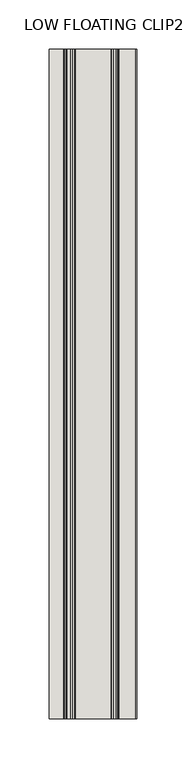
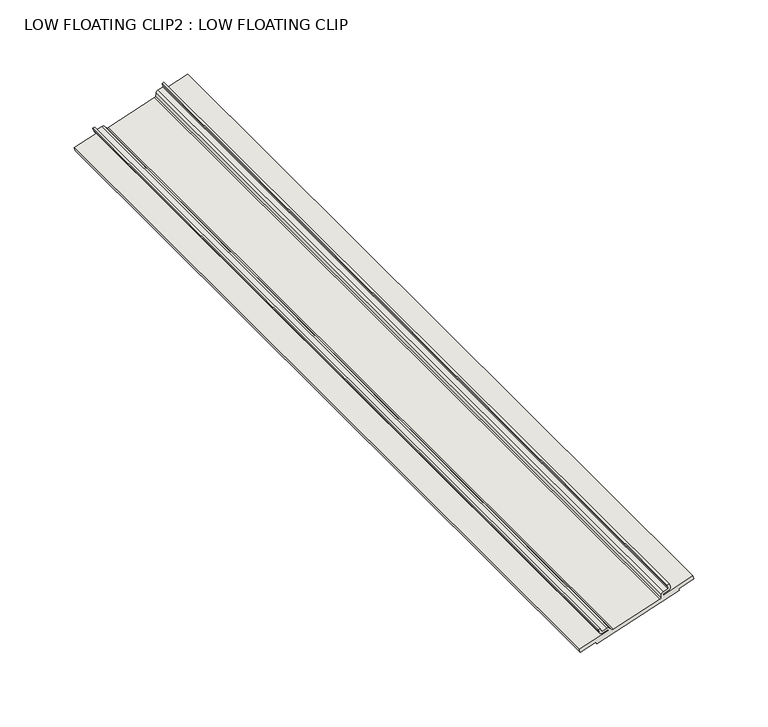
"""IFC4 building model written with IfcOpenShell, lengths in millimetres: wall geometry, LOW FLOATING CLIP2 : LOW FLOATING CLIP."""

from ifc_helpers import new_model, si_unit, frame, origin, place, context, project, spatial, polyline, circle_curve, source, transform, mapped, element, save
from ifc_brep_helpers import plane_surface, cylinder_surface, revolved_surface, advanced_brep


def low_floating_clip2_low_floating_clip_d8918f67(model_context):
    return source(origin(), model_context, "Body", "AdvancedBrep", [
        advanced_brep(
        [(21251.6963274, -2319.6634634, 5817.03297), (21250.2517072, -2319.6634634, 5816.5493228), (21251.0580869, -2319.6634634, 5814.1407232), (21250.6406207, -2319.6634634, 5813.3039581), (21247.0206876, -2319.6634634, 5812.0920337), (21245.5343092, -2319.6634634, 5810.171657), (21245.3411622, -2319.6634634, 5807.4026721), (21244.3180461, -2319.6634634, 5807.060141), (21208.189862, -2319.6634634, 5794.9647155), (21207.1667458, -2319.6634634, 5794.6221844), (21205.3453341, -2319.6634634, 5796.7167113), (21203.0023221, -2319.6634634, 5797.3550388), (21199.3823891, -2319.6634634, 5796.1431143), (21198.5458, -2319.6634634, 5796.5600318), (21197.7388807, -2319.6634634, 5798.9684507), (21196.2942605, -2319.6634634, 5798.4848035), (21197.1006403, -2319.6634634, 5796.076204), (21199.8649785, -2319.6634634, 5794.6985661), (21203.9031762, -2319.6634634, 5796.0505222), (21204.6364349, -2319.6634634, 5795.2073261), (21181.5643102, -2319.6634634, 5787.4829643), (21182.4790038, -2319.6634634, 5784.7508388), (21194.5228505, -2319.6634634, 5788.7830219), (21195.0069954, -2319.6634634, 5787.336915), (21259.436224, -2319.6634634, 5808.9073026), (21258.952079, -2319.6634634, 5810.3534096), (21270.9959257, -2319.6634634, 5814.3855926), (21270.0812321, -2319.6634634, 5817.117718), (21247.0091074, -2319.6634634, 5809.3933561), (21247.0868715, -2319.6634634, 5810.5080761), (21251.1250692, -2319.6634634, 5811.8600323), (21252.5027071, -2319.6634634, 5814.6243705), (21251.6963274, -1637.0384634, 5817.03297), (21252.5027071, -1637.0384634, 5814.6243705), (21251.1250692, -1637.0384634, 5811.8600323), (21247.0868715, -1637.0384634, 5810.5080761), (21247.0091074, -1637.0384634, 5809.3933561), (21270.0812321, -1637.0384634, 5817.117718), (21270.9959257, -1637.0384634, 5814.3855926), (21258.952079, -1637.0384634, 5810.3534096), (21259.436224, -1637.0384634, 5808.9073026), (21195.0069954, -1637.0384634, 5787.336915), (21194.5228505, -1637.0384634, 5788.7830219), (21182.4790038, -1637.0384634, 5784.7508388), (21181.5643102, -1637.0384634, 5787.4829643), (21204.6364349, -1637.0384634, 5795.2073261), (21203.9031762, -1637.0384634, 5796.0505222), (21199.8649785, -1637.0384634, 5794.6985661), (21197.1006403, -1637.0384634, 5796.076204), (21196.2942605, -1637.0384634, 5798.4848035), (21197.7388807, -1637.0384634, 5798.9684507), (21198.5452605, -1637.0384634, 5796.5598512), (21199.3823891, -1637.0384634, 5796.1431143), (21203.0023221, -1637.0384634, 5797.3550388), (21205.3453341, -1637.0384634, 5796.7167113), (21207.1667458, -1637.0384634, 5794.6221844), (21208.189862, -1637.0384634, 5794.9647155), (21244.3180461, -1637.0384634, 5807.060141), (21245.3411622, -1637.0384634, 5807.4026721), (21245.5343092, -1637.0384634, 5810.171657), (21247.0206876, -1637.0384634, 5812.0920337), (21250.6406207, -1637.0384634, 5813.3039581), (21251.0575474, -1637.0384634, 5814.1405426), (21250.2517072, -1637.0384634, 5816.5493228)],
        [
            (0, 1),
            (1, 2),
            (2, 3, circle_curve(frame((21250.4307872, -2319.6634634, 5813.930716), z_axis=(0.0, 1.0, 0.0), x_axis=(0.31747234470250746, 0.0, -0.9482675310001353)), 0.6609505)),
            (3, 4),
            (4, 5, circle_curve(frame((21247.714529, -2319.6634634, 5810.0195786), z_axis=(0.0, -1.0, 0.0), x_axis=(-0.997576050299932, 0.0, 0.06958465253191609)), 2.1855173)),
            (5, 6),
            (6, 7),
            (7, 8),
            (8, 9),
            (9, 10),
            (10, 11, circle_curve(frame((21203.6961634, -2319.6634634, 5795.2825837), z_axis=(0.0, -1.0, 0.0), x_axis=(0.7545905437642736, 0.0, 0.6561959396868727)), 2.1855173)),
            (11, 12),
            (12, 13, circle_curve(frame((21199.1725556, -2319.6634634, 5796.7698722), z_axis=(0.0, 1.0, 0.0), x_axis=(0.3174723447027873, 0.0, -0.9482675310000416)), 0.6609505)),
            (13, 14),
            (14, 15),
            (15, 16),
            (16, 17, circle_curve(frame((21199.1716283, -2319.6634634, 5796.7695541), z_axis=(0.0, -1.0, 0.0), x_axis=(-0.9482675310000763, 0.0, -0.3174723447026833)), 2.1839702)),
            (17, 18),
            (18, 19),
            (19, 20),
            (20, 21),
            (21, 22),
            (22, 23),
            (23, 24),
            (24, 25),
            (25, 26),
            (26, 27),
            (27, 28),
            (28, 29),
            (29, 30),
            (30, 31, circle_curve(frame((21250.4317191, -2319.6634634, 5813.9310203), z_axis=(0.0, -1.0, 0.0), x_axis=(0.9482675310001005, 0.0, 0.31747234470261126)), 2.1839702)),
            (31, 0),
            (32, 33),
            (33, 34, circle_curve(frame((21250.4317191, -1637.0384634, 5813.9310203), z_axis=(0.0, 1.0, 0.0), x_axis=(0.9482675310001005, 0.0, 0.31747234470261126)), 2.1839702)),
            (34, 35),
            (35, 36),
            (36, 37),
            (37, 38),
            (38, 39),
            (39, 40),
            (40, 41),
            (41, 42),
            (42, 43),
            (43, 44),
            (44, 45),
            (45, 46),
            (46, 47),
            (47, 48, circle_curve(frame((21199.1716283, -1637.0384634, 5796.7695541), z_axis=(0.0, 1.0, 0.0), x_axis=(-0.9482675310000763, 0.0, -0.3174723447026833)), 2.1839702)),
            (48, 49),
            (49, 50),
            (50, 51),
            (51, 52, circle_curve(frame((21199.1725556, -1637.0384634, 5796.7698722), z_axis=(0.0, -1.0, 0.0), x_axis=(0.3174723447027873, 0.0, -0.9482675310000416)), 0.6609505)),
            (52, 53),
            (53, 54, circle_curve(frame((21203.6961634, -1637.0384634, 5795.2825837), z_axis=(0.0, 1.0, 0.0), x_axis=(0.7545905437642736, 0.0, 0.6561959396868727)), 2.1855173)),
            (54, 55),
            (55, 56),
            (56, 57),
            (57, 58),
            (58, 59),
            (59, 60, circle_curve(frame((21247.714529, -1637.0384634, 5810.0195786), z_axis=(0.0, 1.0, 0.0), x_axis=(-0.997576050299932, 0.0, 0.06958465253191609)), 2.1855173)),
            (60, 61),
            (61, 62, circle_curve(frame((21250.4307872, -1637.0384634, 5813.930716), z_axis=(0.0, -1.0, 0.0), x_axis=(0.31747234470250746, 0.0, -0.9482675310001353)), 0.6609505)),
            (62, 63),
            (63, 32),
            (31, 33),
            (32, 0),
            (30, 34),
            (29, 35),
            (28, 36),
            (27, 37),
            (26, 38),
            (25, 39),
            (24, 40),
            (23, 41),
            (22, 42),
            (21, 43),
            (20, 44),
            (19, 45),
            (18, 46),
            (17, 47),
            (16, 48),
            (15, 49),
            (14, 50),
            (13, 51),
            (12, 52),
            (11, 53),
            (10, 54),
            (9, 55),
            (8, 56),
            (7, 57),
            (6, 58),
            (5, 59),
            (4, 60),
            (3, 61),
            (2, 62),
            (1, 63),
        ],
        [
            plane_surface(frame((21250.2511677, -2319.6634634, 5816.5491422), z_axis=(0.0, -1.0000000000000002, 0.0), x_axis=(-0.9482675310000759, 0.0, -0.3174723447026848))),
            plane_surface(frame((21250.2511677, -1637.0384634, 5816.5491422), z_axis=(0.0, 1.0000000000000002, 0.0), x_axis=(0.9482675310000759, 0.0, 0.3174723447026848))),
            plane_surface(frame((21252.5027071, -2319.6634634, 5814.6243705), z_axis=(0.9482675310001323, 0.0, 0.3174723447025162), x_axis=(0.0, 1.0, 0.0))),
            cylinder_surface(frame((21250.4317191, -1637.0384634, 5813.9310203), z_axis=(0.0, -1.0000000000000002, 0.0), x_axis=(0.9482675310001005, 0.0, 0.31747234470261126)), 2.1839702),
            plane_surface(frame((21247.0868715, -2319.6634634, 5810.5080761), z_axis=(0.3174723445422707, 0.0, -0.9482675310537811), x_axis=(0.0, 1.0, 0.0))),
            plane_surface(frame((21247.0091074, -2319.6634634, 5809.3933561), z_axis=(0.9975755390756385, 0.0, -0.06959198113252213), x_axis=(0.0, 1.0, 0.0))),
            plane_surface(frame((21270.0812321, -2319.6634634, 5817.117718), z_axis=(-0.3174723447025733, 0.0, 0.9482675310001131), x_axis=(0.0, 1.0, 0.0))),
            plane_surface(frame((21270.9959257, -2319.6634634, 5814.3855926), z_axis=(0.9482675310001432, 0.0, 0.3174723447024835), x_axis=(0.0, 1.0, 0.0))),
            plane_surface(frame((21258.952079, -2319.6634634, 5810.3534096), z_axis=(0.3174723447026279, 0.0, -0.9482675310000949), x_axis=(0.0, 1.0, 0.0))),
            plane_surface(frame((21259.436224, -2319.6634634, 5808.9073026), z_axis=(0.9482675310001084, 0.0, 0.31747234470258734), x_axis=(0.0, 1.0, 0.0))),
            plane_surface(frame((21195.0069954, -2319.6634634, 5787.336915), z_axis=(0.31747234470254, 0.0, -0.9482675310001243), x_axis=(0.0, 1.0, 0.0))),
            plane_surface(frame((21194.5228505, -2319.6634634, 5788.7830219), z_axis=(-0.9482675310005341, 0.0, -0.3174723447013159), x_axis=(0.0, 1.0, 0.0))),
            plane_surface(frame((21182.4790038, -2319.6634634, 5784.7508388), z_axis=(0.3174723447026786, 0.0, -0.9482675310000779), x_axis=(0.0, 1.0, 0.0))),
            plane_surface(frame((21181.5643102, -2319.6634634, 5787.4829643), z_axis=(-0.9482675310000674, 0.0, -0.31747234470270974), x_axis=(0.0, 1.0, 0.0))),
            plane_surface(frame((21204.6364349, -2319.6634634, 5795.2073261), z_axis=(-0.31747234470271984, 0.0, 0.9482675310000641), x_axis=(0.0, 1.0, 0.0))),
            plane_surface(frame((21203.9031762, -2319.6634634, 5796.0505222), z_axis=(-0.7545857230581579, 0.0, -0.6562014832022228), x_axis=(0.0, 1.0, 0.0))),
            plane_surface(frame((21199.8649785, -2319.6634634, 5794.6985661), z_axis=(0.3174723447025522, 0.0, -0.9482675310001202), x_axis=(0.0, 1.0, 0.0))),
            cylinder_surface(frame((21199.1716283, -1637.0384634, 5796.7695541), z_axis=(0.0, -1.0, 0.0), x_axis=(-0.9482675310000763, 0.0, -0.3174723447026833)), 2.1839702),
            plane_surface(frame((21196.2942605, -2319.6634634, 5798.4848035), z_axis=(-0.9482675309984633, 0.0, -0.31747234470750146), x_axis=(0.0, 1.0, 0.0))),
            plane_surface(frame((21197.7388807, -2319.6634634, 5798.9684507), z_axis=(-0.3174723447029016, 0.0, 0.9482675310000033), x_axis=(0.0, 1.0, 0.0))),
            plane_surface(frame((21198.5452605, -2319.6634634, 5796.5598512), z_axis=(0.9482675310001752, 0.0, 0.31747234470238783), x_axis=(0.0, 1.0, 0.0))),
            revolved_surface(polyline([(21199.382389104965, -1637.0384634, 5796.143114301251), (21199.382389104965, -2319.6634634, 5796.143114301251)]), (21199.1725556, -1637.0384634, 5796.7698722), (0.0, 1.0000000000000002, 0.0)),
            plane_surface(frame((21203.0023221, -2319.6634634, 5797.3550388), z_axis=(-0.31747234470292157, 0.0, 0.9482675309999966), x_axis=(0.0, 1.0, 0.0))),
            cylinder_surface(frame((21203.6961634, -1637.0384634, 5795.2825837), z_axis=(0.0, -1.0000000000000002, 0.0), x_axis=(0.7545905437642736, 0.0, 0.6561959396868727)), 2.1855173),
            plane_surface(frame((21207.1667458, -2319.6634634, 5794.6221844), z_axis=(0.7545905437681126, 0.0, 0.656195939682458), x_axis=(0.0, 1.0, 0.0))),
            plane_surface(frame((21208.189862, -2319.6634634, 5794.9647155), z_axis=(-0.31747234470267577, 0.0, 0.9482675310000789), x_axis=(0.0, 1.0, 0.0))),
            plane_surface(frame((21244.3180461, -2319.6634634, 5807.060141), z_axis=(-0.3174723447026769, 0.0, 0.9482675310000784), x_axis=(0.0, 1.0, 0.0))),
            plane_surface(frame((21245.3411622, -2319.6634634, 5807.4026721), z_axis=(-0.31747234470207936, 0.0, 0.9482675310002785), x_axis=(0.0, 1.0, 0.0))),
            plane_surface(frame((21245.5343092, -2319.6634634, 5810.171657), z_axis=(-0.9975760502999373, 0.0, 0.06958465253183929), x_axis=(0.0, 1.0, 0.0))),
            cylinder_surface(frame((21247.714529, -1637.0384634, 5810.0195786), z_axis=(0.0, -1.0, 0.0), x_axis=(-0.997576050299932, 0.0, 0.06958465253191609)), 2.1855173),
            plane_surface(frame((21250.6406207, -2319.6634634, 5813.3039581), z_axis=(-0.317472342372389, 0.0, 0.9482675317802401), x_axis=(0.0, 1.0, 0.0))),
            revolved_surface(polyline([(21250.640620704966, -1637.0384634, 5813.303958101252), (21250.640620704966, -2319.6634634, 5813.303958101252)]), (21250.4307872, -1637.0384634, 5813.930716), (0.0, 1.0000000000000002, 0.0)),
            plane_surface(frame((21250.2517072, -2319.6634634, 5816.5493228), z_axis=(-0.9482675310001136, 0.0, -0.3174723447025722), x_axis=(0.0, 1.0, 0.0))),
            plane_surface(frame((21251.6963274, -2319.6634634, 5817.03297), z_axis=(-0.3174723447026848, 0.0, 0.9482675310000759), x_axis=(0.0, 1.0, 0.0))),
        ],
        [
            (0, [[1, 2, 3, 4, 5, 6, 7, 8, 9, 10, 11, 12, 13, 14, 15, 16, 17, 18, 19, 20, 21, 22, 23, 24, 25, 26, 27, 28, 29, 30, 31, 32]]),
            (1, [[33, 34, 35, 36, 37, 38, 39, 40, 41, 42, 43, 44, 45, 46, 47, 48, 49, 50, 51, 52, 53, 54, 55, 56, 57, 58, 59, 60, 61, 62, 63, 64]]),
            (2, [[-32, 65, -33, 66]]),
            (3, [[-31, 67, -34, -65]]),
            (4, [[-30, 68, -35, -67]]),
            (5, [[-29, 69, -36, -68]]),
            (6, [[-28, 70, -37, -69]]),
            (7, [[-27, 71, -38, -70]]),
            (8, [[-26, 72, -39, -71]]),
            (9, [[-25, 73, -40, -72]]),
            (10, [[-24, 74, -41, -73]]),
            (11, [[-23, 75, -42, -74]]),
            (12, [[-22, 76, -43, -75]]),
            (13, [[-21, 77, -44, -76]]),
            (14, [[-20, 78, -45, -77]]),
            (15, [[-19, 79, -46, -78]]),
            (16, [[-18, 80, -47, -79]]),
            (17, [[-17, 81, -48, -80]]),
            (18, [[-16, 82, -49, -81]]),
            (19, [[-15, 83, -50, -82]]),
            (20, [[-14, 84, -51, -83]]),
            (21, [[-13, 85, -52, -84]]),
            (22, [[-12, 86, -53, -85]]),
            (23, [[-11, 87, -54, -86]]),
            (24, [[-10, 88, -55, -87]]),
            (25, [[-9, 89, -56, -88]]),
            (26, [[-8, 90, -57, -89]]),
            (27, [[-7, 91, -58, -90]]),
            (28, [[-6, 92, -59, -91]]),
            (29, [[-5, 93, -60, -92]]),
            (30, [[-4, 94, -61, -93]]),
            (31, [[-3, 95, -62, -94]]),
            (32, [[-2, 96, -63, -95]]),
            (33, [[-1, -66, -64, -96]]),
        ],
    ),
    ])


if __name__ == "__main__":
    model = new_model("IFC4")
    model_context = context("Model", 3, world=origin())
    ifc_project = project(units=[si_unit("LENGTHUNIT", "METRE", prefix="MILLI")], contexts=[model_context])
    site = spatial("IfcSite", under=ifc_project)
    building = spatial("IfcBuilding", under=site)
    placement = place(None, origin())
    low_floating_clip2_low_floating_clip_shape = low_floating_clip2_low_floating_clip_d8918f67(model_context)
    element("IfcWall", 1, ObjectType="LOW FLOATING CLIP2 : LOW FLOATING CLIP", at=placement, inside=building, context=model_context, shape_type="MappedRepresentation", body=[
        mapped(low_floating_clip2_low_floating_clip_shape, transform((0.0, 0.0, 0.0), x_axis=(1.0, 0.0, 0.0), y_axis=(0.0, 1.0, 0.0), z_axis=(0.0, 0.0, 1.0))),
    ])
    save(model, "model.ifc")

# Revit data of these elements
# Element 1 (IfcWall, "LOW FLOATING CLIP2 : LOW FLOATING CLIP")
#   Materials on its faces: "LOW FLOATING CLIP"
# Materials
#   "LOW FLOATING CLIP": class "Metal", colour RGB 247 247 247, transparency 0, Cost = 0
